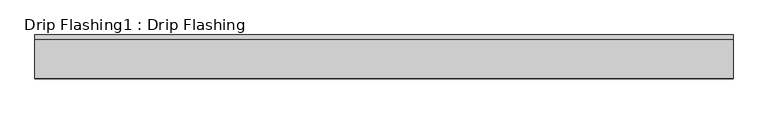
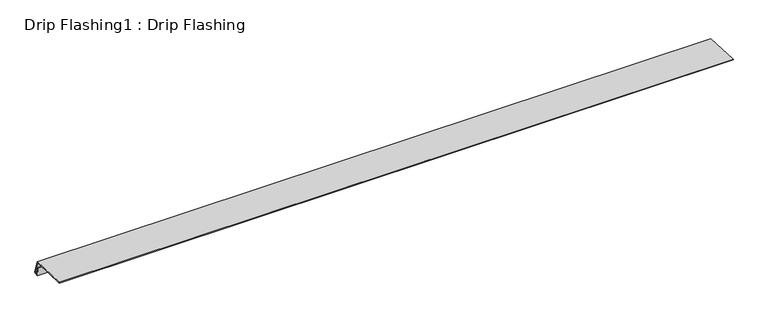
"""IFC4 building model written with IfcOpenShell, lengths in millimetres: proxy geometry, Drip Flashing1 : Drip Flashing."""

from ifc_helpers import new_model, si_unit, frame, origin, place, context, project, spatial, polyline, outline, extrude, source, transform, mapped, element, save


def drip_flashing1_drip_flashing_05063a31(model_context):
    return source(origin(), model_context, "Body", "SweptSolid", [
        extrude(outline(polyline([(9772.4316207, 37600.241418), (9660.1127629, 37604.8160522), (9660.1989012, 37606.9309658), (9774.0264732, 37602.2948832), (9786.1199219, 37561.887738), (9774.040701, 37558.2725497), (9771.4197382, 37583.2093446), (9773.5082342, 37583.4288544), (9775.8645053, 37561.0104321), (9783.490007, 37563.2926674), (9772.4316207, 37600.241418)])), frame((-9232.0719278, 0.0, 0.0), z_axis=(1.0, 0.0, 0.0), x_axis=(0.0, 1.0, 0.0)), (0.0, 0.0, 1.0), 1999.85),
    ])


if __name__ == "__main__":
    model = new_model("IFC4")
    model_context = context("Model", 3, world=origin())
    ifc_project = project(units=[si_unit("LENGTHUNIT", "METRE", prefix="MILLI")], contexts=[model_context])
    site = spatial("IfcSite", under=ifc_project)
    building = spatial("IfcBuilding", under=site)
    placement = place(None, origin())
    drip_flashing1_drip_flashing_shape = drip_flashing1_drip_flashing_05063a31(model_context)
    element("IfcBuildingElementProxy", 1, Name="Drip Flashing1 : Drip Flashing", ObjectType="Drip Flashing1 : Drip Flashing", at=placement, inside=building, context=model_context, shape_type="MappedRepresentation", body=[
        mapped(drip_flashing1_drip_flashing_shape, transform((0.0, 0.0, 0.0), x_axis=(1.0, 0.0, 0.0), y_axis=(0.0, 1.0, 0.0), z_axis=(0.0, 0.0, 1.0))),
    ])
    save(model, "model.ifc")

# Revit data of these elements
# Type "Drip Flashing1 : Drip Flashing"
#   NameOverride = "Drip Flashing"
# Element 1 (IfcBuildingElementProxy, "Drip Flashing1 : Drip Flashing")
#   Materials on its faces: "16 GA. COPPER BRAKE METAL FLASHING"
# Materials
#   "16 GA. COPPER BRAKE METAL FLASHING": class "Unassigned", colour RGB 128 128 128, transparency 0
